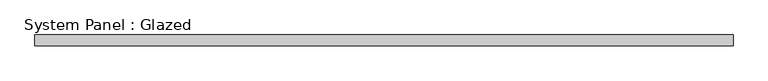
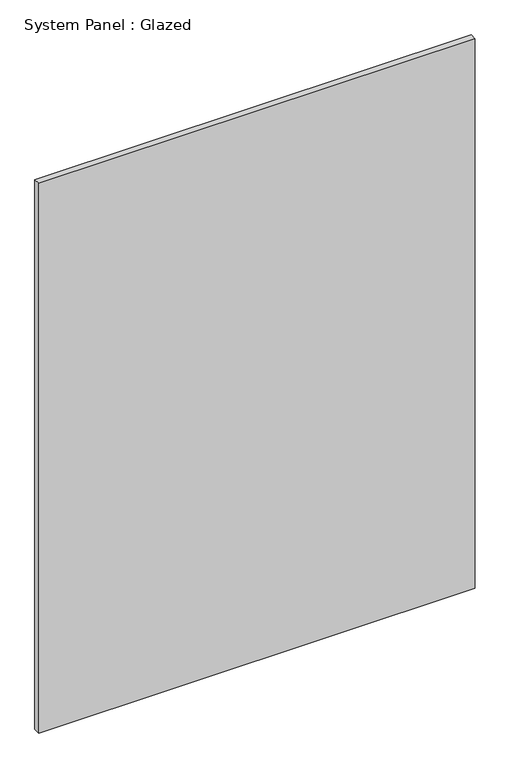
"""IFC4 building model written with IfcOpenShell, lengths in millimetres: plate geometry, System Panel : Glazed."""

from ifc_helpers import new_model, si_unit, origin, origin_with_axes, place, context, project, spatial, polyline, outline, extrude, source, transform, mapped, element, save


def system_panel_glazed_3d35191a(model_context):
    return source(origin(), model_context, "Body", "SweptSolid", [
        extrude(outline(polyline([(807.775, -49.5), (-807.775, -49.5), (-807.775, -24.5), (807.775, -24.5), (807.775, -49.5)])), origin_with_axes(), (0.0, 0.0, 1.0), 2150.0),
    ])


if __name__ == "__main__":
    model = new_model("IFC4")
    model_context = context("Model", 3, world=origin())
    ifc_project = project(units=[si_unit("LENGTHUNIT", "METRE", prefix="MILLI")], contexts=[model_context])
    site = spatial("IfcSite", under=ifc_project)
    building = spatial("IfcBuilding", under=site)
    placement = place(None, origin())
    system_panel_glazed_shape = system_panel_glazed_3d35191a(model_context)
    element("IfcPlate", 1, ObjectType="System Panel : Glazed", at=placement, inside=building, context=model_context, shape_type="MappedRepresentation", body=[
        mapped(system_panel_glazed_shape, transform((0.0, 0.0, 0.0), x_axis=(1.0, 0.0, 0.0), y_axis=(0.0, 1.0, 0.0), z_axis=(0.0, 0.0, 1.0))),
    ])
    save(model, "model.ifc")

# Revit data of these elements
# Type "System Panel : Glazed"
#   Keynote = "H11"
#   Construction Type Id = "GSP4R"
#   Analytic Construction = "1/8 in Pilkington single glazing"
#   Visual Light Transmittance = 0.9
#   Solar Heat Gain Coefficient = 0.86
#   Heat Transfer Coefficient (U) = 6.7069 W/(m²·K)
# Element 1 (IfcPlate, "System Panel : Glazed")
#   Materials on its faces: "Glass"
# Materials
#   "Glass": class "Glass", colour RGB 0 128 192, transparency 0.9, Description = "Soda Lime Glass", Cost = 0
